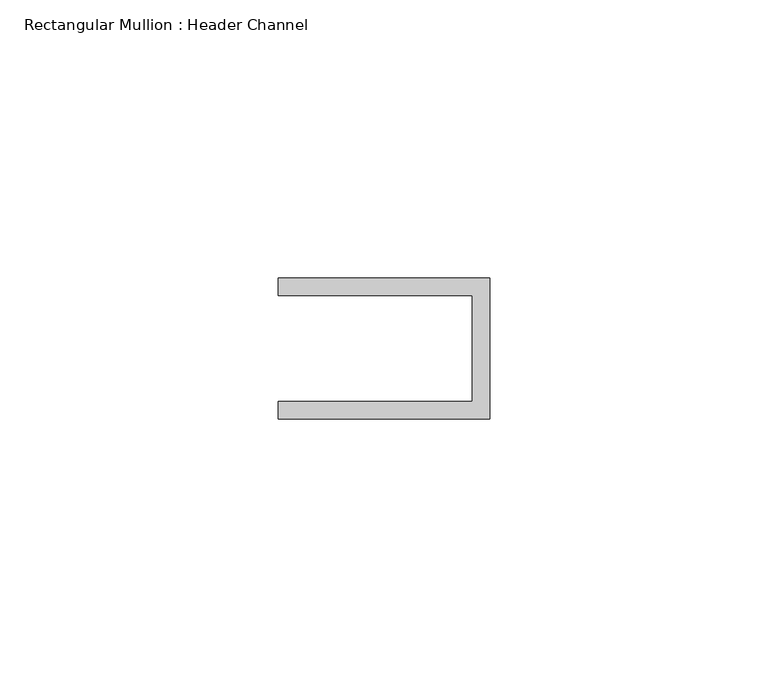
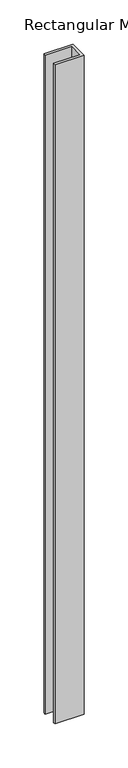
"""IFC4 building model written with IfcOpenShell, lengths in millimetres: member geometry, Rectangular Mullion : Header Channel."""

from ifc_helpers import new_model, si_unit, frame, origin, place, context, project, spatial, polyline, outline, extrude, source, transform, mapped, element, save


def rectangular_mullion_header_channel_60ad953d(model_context):
    return source(origin(), model_context, "Body", "SweptSolid", [
        extrude(outline(polyline([(0.0, -12.7), (-38.1, -12.7), (-38.1, -9.525), (-3.175, -9.525), (-3.175, 9.525), (-38.1, 9.525), (-38.1, 12.7), (0.0, 12.7), (0.0, -12.7)])), frame((0.0, 0.0, -914.3999999), z_axis=(0.0, 0.0, 1.0), x_axis=(1.0, 0.0, 0.0)), (0.0, 0.0, 1.0), 914.3999999),
    ])


if __name__ == "__main__":
    model = new_model("IFC4")
    model_context = context("Model", 3, world=origin())
    ifc_project = project(units=[si_unit("LENGTHUNIT", "METRE", prefix="MILLI")], contexts=[model_context])
    site = spatial("IfcSite", under=ifc_project)
    building = spatial("IfcBuilding", under=site)
    placement = place(None, origin())
    rectangular_mullion_header_channel_shape = rectangular_mullion_header_channel_60ad953d(model_context)
    element("IfcMember", 1, ObjectType="Rectangular Mullion : Header Channel", at=placement, inside=building, context=model_context, shape_type="MappedRepresentation", body=[
        mapped(rectangular_mullion_header_channel_shape, transform((0.0, 0.0, 0.0), x_axis=(1.0, 0.0, 0.0), y_axis=(0.0, 1.0, 0.0), z_axis=(0.0, 0.0, 1.0))),
    ])
    save(model, "model.ifc")

# Revit data of these elements
# Type "Rectangular Mullion : Header Channel"
#   built-in parameter 1007322 = 0.0833333 (stored number, unit not read)
#   built-in parameter 1007321 = -0.03125 (stored number, unit not read)
#   built-in parameter 1007320 = 0.0416667 (stored number, unit not read)
# Element 1 (IfcMember, "Rectangular Mullion : Header Channel")
#   Materials on its faces: "ALUM"
# Materials
#   "ALUM": class "Generic", colour RGB 157 157 157, transparency 0, Cost = 0
